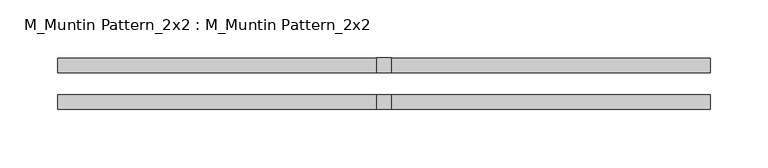
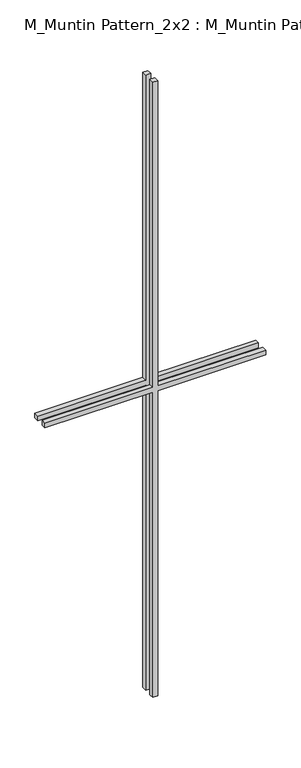
"""IFC4 building model written with IfcOpenShell, lengths in millimetres: proxy geometry, M_Muntin Pattern_2x2 : M_Muntin Pattern_2x2."""

import ifcopenshell
import ifcopenshell.guid

model = None  # the IFC model being written
_history = None  # IfcOwnerHistory: only IFC2X3 demands one
_inside = {}  # id of a spatial element -> (the spatial element, [elements in it])
_under = {}  # id of a project, library or spatial element -> (it, [spatial elements below it])
_declared = {}  # id of a project -> (the project, [libraries it declares])
_typed = {}  # id of a type object -> (the type object, [elements of that type])
_made_of = {}  # id of a material, layer set ... -> (it, [elements and type objects made of it])


def new_model(schema):
    """Start an empty IFC model of exactly this schema.

    Asked for "IFC4X3", IfcOpenShell would pick the latest addendum, in which some entities
    have other attributes; the version numbers below select the first issue.
    IFC2X3 requires an IfcOwnerHistory on every rooted entity: one is made here for all.
    """
    global model, _history
    if schema == "IFC4X3":
        model = ifcopenshell.file(schema_version=(4, 3, 0, 0))
    else:
        model = ifcopenshell.file(schema=schema)
    _inside.clear()
    _under.clear()
    _declared.clear()
    _typed.clear()
    _made_of.clear()
    _history = None
    if model.schema == "IFC2X3":
        org = make("IfcOrganization", Name="unknown")
        user = make(
            "IfcPersonAndOrganization",
            ThePerson=make("IfcPerson", FamilyName="unknown"),
            TheOrganization=org,
        )
        app = make(
            "IfcApplication",
            ApplicationDeveloper=org,
            Version="unknown",
            ApplicationFullName="unknown",
            ApplicationIdentifier="unknown",
        )
        _history = make(
            "IfcOwnerHistory",
            OwningUser=user,
            OwningApplication=app,
            ChangeAction="ADDED",
            CreationDate=0,
        )
    return model


def make(cls, **values):
    """One entity of the class cls with the attributes given. An attribute that is None is left unset."""
    return model.create_entity(
        cls, **{name: value for name, value in values.items() if value is not None}
    )


def rooted(cls, **values):
    """An entity with a GlobalId (a new one), such as an element, a storey or a relation."""
    return make(cls, GlobalId=ifcopenshell.guid.new(), OwnerHistory=_history, **values)


def si_unit(unit_type, name, prefix=None):
    """IfcSIUnit, for example si_unit("LENGTHUNIT", "METRE", prefix="MILLI")."""
    return make("IfcSIUnit", UnitType=unit_type, Prefix=prefix, Name=name)


def assignment(units):
    """IfcUnitAssignment: the units of a project."""
    return None if units is None else make("IfcUnitAssignment", Units=units)


def point(xyz):
    """IfcCartesianPoint."""
    return None if xyz is None else make("IfcCartesianPoint", Coordinates=xyz)


def direction(xyz):
    """IfcDirection."""
    return None if xyz is None else make("IfcDirection", DirectionRatios=xyz)


def frame(location, z_axis=None, x_axis=None):
    """IfcAxis2Placement3D, a coordinate frame: its origin and axes. An axis left out is left unset."""
    return make(
        "IfcAxis2Placement3D",
        Location=point(location),
        Axis=direction(z_axis),
        RefDirection=direction(x_axis),
    )


def origin():
    """The frame at (0, 0, 0) with its axes left unset."""
    return frame((0.0, 0.0, 0.0))


def place(relative_to, where):
    """IfcLocalPlacement: puts the frame where relative to a parent placement (None: the world)."""
    return make(
        "IfcLocalPlacement", PlacementRelTo=relative_to, RelativePlacement=where
    )


def context(
    kind, dimensions, precision=None, world=None, true_north=None, identifier=None
):
    """IfcGeometricRepresentationContext, for example the 3D "Model" context."""
    return make(
        "IfcGeometricRepresentationContext",
        ContextIdentifier=identifier,
        ContextType=kind,
        CoordinateSpaceDimension=dimensions,
        Precision=precision,
        WorldCoordinateSystem=world,
        TrueNorth=true_north,
    )


def project(units=None, contexts=None):
    """IfcProject with its units and contexts."""
    return rooted(
        "IfcProject",
        Name="project",
        RepresentationContexts=contexts,
        UnitsInContext=assignment(units),
    )


def spatial(cls, under=None, at=None, **own):
    """A site, building, storey or space (cls), placed at a placement, below another one or the project."""
    s = rooted(cls, ObjectPlacement=at, **own)
    if under is not None:
        _under.setdefault(under.id(), (under, []))[1].append(s)
    return s


def polyline(points):
    """IfcPolyline through the points."""
    return make("IfcPolyline", Points=[point(p) for p in points])


def outline(outer, holes=None, kind="AREA"):
    """IfcArbitraryClosedProfileDef: a profile drawn as a closed curve; with holes, ...WithVoids."""
    if holes is None:
        return make("IfcArbitraryClosedProfileDef", ProfileType=kind, OuterCurve=outer)
    return make(
        "IfcArbitraryProfileDefWithVoids",
        ProfileType=kind,
        OuterCurve=outer,
        InnerCurves=holes,
    )


def extrude(swept, where, along, depth):
    """IfcExtrudedAreaSolid: the profile swept, set in the frame where, extruded along a direction by depth."""
    return make(
        "IfcExtrudedAreaSolid",
        SweptArea=swept,
        Position=where,
        ExtrudedDirection=direction(along),
        Depth=depth,
    )


def shape(context_of_items, identifier, shape_type, items):
    """IfcShapeRepresentation: the items that make up one representation, for example the "Body"."""
    return make(
        "IfcShapeRepresentation",
        ContextOfItems=context_of_items,
        RepresentationIdentifier=identifier,
        RepresentationType=shape_type,
        Items=items,
    )


def source(mapping_origin, context_of_items, identifier, shape_type, items):
    """IfcRepresentationMap: a shape defined once, which mapped items show again and again."""
    return make(
        "IfcRepresentationMap",
        MappingOrigin=mapping_origin,
        MappedRepresentation=shape(context_of_items, identifier, shape_type, items),
    )


def transform(
    local_origin,
    x_axis=None,
    y_axis=None,
    z_axis=None,
    scale=None,
    scale2=None,
    scale3=None,
    uniform=True,
):
    """IfcCartesianTransformationOperator3D, or its non-uniform kind. x_axis, y_axis, z_axis: its Axis1, 2, 3."""
    if uniform:
        return make(
            "IfcCartesianTransformationOperator3D",
            Axis1=direction(x_axis),
            Axis2=direction(y_axis),
            LocalOrigin=point(local_origin),
            Scale=scale,
            Axis3=direction(z_axis),
        )
    return make(
        "IfcCartesianTransformationOperator3DnonUniform",
        Axis1=direction(x_axis),
        Axis2=direction(y_axis),
        LocalOrigin=point(local_origin),
        Scale=scale,
        Axis3=direction(z_axis),
        Scale2=scale2,
        Scale3=scale3,
    )


def mapped(mapping_source, mapping_target):
    """IfcMappedItem: shows the shape of a source again, moved by a transform."""
    return make(
        "IfcMappedItem", MappingSource=mapping_source, MappingTarget=mapping_target
    )


def made_of(thing, what):
    """Note that an element or type object is made of a material, layer set ...; save() writes the relation."""
    if what is not None:
        _made_of.setdefault(what.id(), (what, []))[1].append(thing)
    return thing


def element(
    cls,
    number,
    at=None,
    inside=None,
    cuts=None,
    type_object=None,
    material=None,
    context=None,
    identifier="Body",
    shape_type=None,
    held_by="IfcProductDefinitionShape",
    body=None,
    shapes=None,
    **own,
):
    """One element of the class cls, such as IfcWall. Its Tag is "e" and its number.

    at: its placement. inside: the storey or other place that contains it. cuts: it is an
    opening in that element (IfcRelVoidsElement). A single representation is given by context,
    identifier, shape_type and body (its items); several are given by shapes. held_by: the class
    of the entity that holds the representations. save() writes the other relations.
    """
    e = rooted(cls, Tag="e%d" % number, ObjectPlacement=at, **own)
    if body is not None:
        shapes = [shape(context, identifier, shape_type, body)]
    if shapes is not None:
        e.Representation = make(held_by, Representations=shapes)
    if inside is not None:
        _inside.setdefault(inside.id(), (inside, []))[1].append(e)
    if cuts is not None:
        rooted(
            "IfcRelVoidsElement", RelatingBuildingElement=cuts, RelatedOpeningElement=e
        )
    if type_object is not None:
        _typed.setdefault(type_object.id(), (type_object, []))[1].append(e)
    return made_of(e, material)


def aggregate(whole, parts):
    """IfcRelAggregates: a whole, such as a stair, and the parts it consists of."""
    return rooted("IfcRelAggregates", RelatingObject=whole, RelatedObjects=parts)


def save(model, path):
    """Write the relations noted so far, then the file.

    IfcRelAggregates (storeys below a building ...), IfcRelContainedInSpatialStructure (elements
    in a storey), IfcRelDefinesByType, IfcRelAssociatesMaterial and IfcRelDeclares: one each for
    every whole, place, type object, material and project.
    """
    for whole, parts in _under.values():
        aggregate(whole, parts)
    for where, things in _inside.values():
        rooted(
            "IfcRelContainedInSpatialStructure",
            RelatedElements=things,
            RelatingStructure=where,
        )
    for kind, things in _typed.values():
        rooted("IfcRelDefinesByType", RelatedObjects=things, RelatingType=kind)
    for what, things in _made_of.values():
        rooted("IfcRelAssociatesMaterial", RelatedObjects=things, RelatingMaterial=what)
    for by, libraries in _declared.values():
        rooted("IfcRelDeclares", RelatingContext=by, RelatedDefinitions=libraries)
    model.write(path)


def m_muntin_pattern_2x2_m_muntin_pattern_2x2_f3921bb5(model_context):
    return source(origin(), model_context, "Body", "SweptSolid", [
        extrude(outline(polyline([(836.5, -6.35), (836.5, -281.7375), (823.8, -281.7375), (823.8, -6.35), (0.0, -6.35), (0.0, 6.35), (823.8, 6.35), (823.8, 281.7375), (836.5, 281.7375), (836.5, 6.35), (1660.3, 6.35), (1660.3, -6.35), (836.5, -6.35)])), frame((0.0, -22.225, 0.0), z_axis=(0.0, 1.0, 0.0), x_axis=(0.0, 0.0, 1.0)), (0.0, 0.0, 1.0), 12.7),
        extrude(outline(polyline([(836.5, -6.35), (836.5, -281.7375), (823.8, -281.7375), (823.8, -6.35), (0.0, -6.35), (0.0, 6.35), (823.8, 6.35), (823.8, 281.7375), (836.5, 281.7375), (836.5, 6.35), (1660.3, 6.35), (1660.3, -6.35), (836.5, -6.35)])), frame((0.0, 9.525, 0.0), z_axis=(0.0, 1.0, 0.0), x_axis=(0.0, 0.0, 1.0)), (0.0, 0.0, 1.0), 12.7),
    ])


if __name__ == "__main__":
    model = new_model("IFC4")
    model_context = context("Model", 3, world=origin())
    ifc_project = project(units=[si_unit("LENGTHUNIT", "METRE", prefix="MILLI")], contexts=[model_context])
    site = spatial("IfcSite", under=ifc_project)
    building = spatial("IfcBuilding", under=site)
    placement = place(None, origin())
    m_muntin_pattern_2x2_m_muntin_pattern_2x2_shape = m_muntin_pattern_2x2_m_muntin_pattern_2x2_f3921bb5(model_context)
    element("IfcBuildingElementProxy", 1, Name="M_Muntin Pattern_2x2 : M_Muntin Pattern_2x2", ObjectType="M_Muntin Pattern_2x2 : M_Muntin Pattern_2x2", at=placement, inside=building, context=model_context, shape_type="MappedRepresentation", body=[
        mapped(m_muntin_pattern_2x2_m_muntin_pattern_2x2_shape, transform((0.0, 0.0, 0.0), x_axis=(1.0, 0.0, 0.0), y_axis=(0.0, 1.0, 0.0), z_axis=(0.0, 0.0, 1.0))),
    ])
    save(model, "model.ifc")

# Revit data of these elements
# Type "M_Muntin Pattern_2x2 : M_Muntin Pattern_2x2"
#   Width [instance default] = 1200 mm
#   Thickness = 12.7 mm
#   Height [instance default] = 1200 mm
#   Distance = 19.05 mm
#   Interior Material [instance default] = none
#   Exterior Material [instance default] = none
#   Default Elevation = 0
# Element 1 (IfcBuildingElementProxy, "M_Muntin Pattern_2x2 : M_Muntin Pattern_2x2")
#   Width = 563.475 mm
#   Height = 1660.3 mm
#   Interior Material = Wood - Stained
#   Exterior Material = Clad - White
#   Materials on its faces: "Clad - White", "Wood - Stained"
# Materials
#   "Clad - White": class "Wood", colour RGB 245 245 243, transparency 0, Cost = 0
#   "Wood - Stained": class "Wood", colour RGB 173 132 96, transparency 0, Cost = 0
